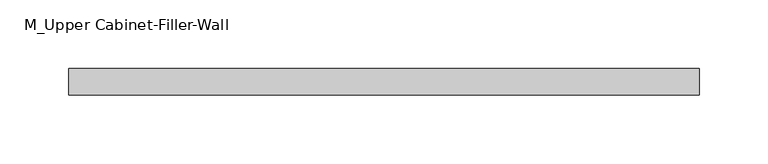
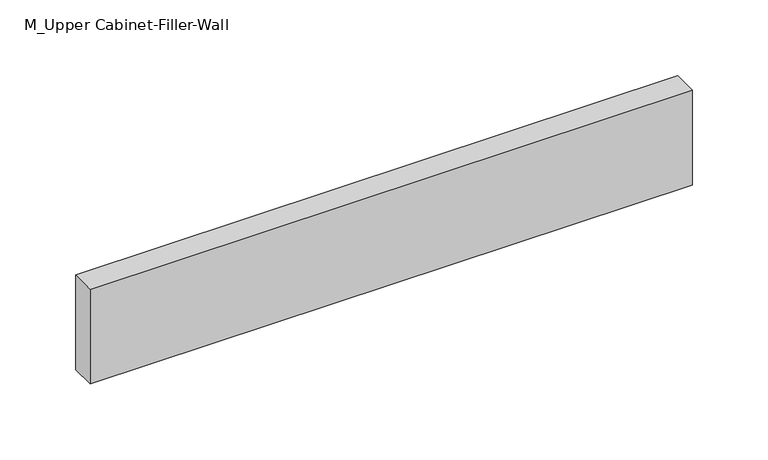
"""IFC4 building model written with IfcOpenShell, lengths in millimetres: furniture geometry, M_Upper Cabinet-Filler-Wall : fhorizontal1."""

from ifc_helpers import new_model, si_unit, frame, origin, place, context, project, spatial, polyline, outline, extrude, source, transform, mapped, element, save


def m_upper_cabinet_filler_wall_65b3d82e(model_context):
    return source(origin(), model_context, "Body", "SweptSolid", [
        extrude(outline(polyline([(-198.8288372, 38.1), (-198.8288372, 57.15), (258.3711628, 57.15), (258.3711628, 38.1), (-198.8288372, 38.1)])), frame((0.0, 0.0, 1923.8), z_axis=(0.0, 0.0, 1.0), x_axis=(1.0, 0.0, 0.0)), (0.0, 0.0, 1.0), 76.2),
    ])


if __name__ == "__main__":
    model = new_model("IFC4")
    model_context = context("Model", 3, world=origin())
    ifc_project = project(units=[si_unit("LENGTHUNIT", "METRE", prefix="MILLI")], contexts=[model_context])
    site = spatial("IfcSite", under=ifc_project)
    building = spatial("IfcBuilding", under=site)
    placement = place(None, origin())
    m_upper_cabinet_filler_wall_shape = m_upper_cabinet_filler_wall_65b3d82e(model_context)
    element("IfcFurniture", 1, ObjectType="M_Upper Cabinet-Filler-Wall : fhorizontal1", at=placement, inside=building, context=model_context, shape_type="MappedRepresentation", body=[
        mapped(m_upper_cabinet_filler_wall_shape, transform((0.0, 0.0, 0.0), x_axis=(1.0, 0.0, 0.0), y_axis=(0.0, 1.0, 0.0), z_axis=(0.0, 0.0, 1.0))),
    ])
    save(model, "model.ifc")

# Revit data of these elements
# Type "M_Upper Cabinet-Filler-Wall : fhorizontal1"
#   Depth = 0' - 1"
#   Height = 0' - 3"
#   Top Of Cabinet = 6' - 6.74016"
#   Width = 1' - 6"
#   Cabinet Material = none
#   Default Elevation = 0
# Element 1 (IfcFurniture, "M_Upper Cabinet-Filler-Wall : fhorizontal1")
#   Materials on its faces: "Cabinets"
# Materials
#   "Cabinets": class "Miscellaneous", colour RGB 249 249 249, transparency 0
